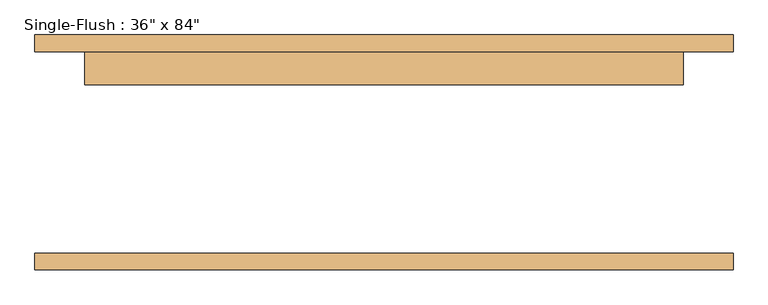
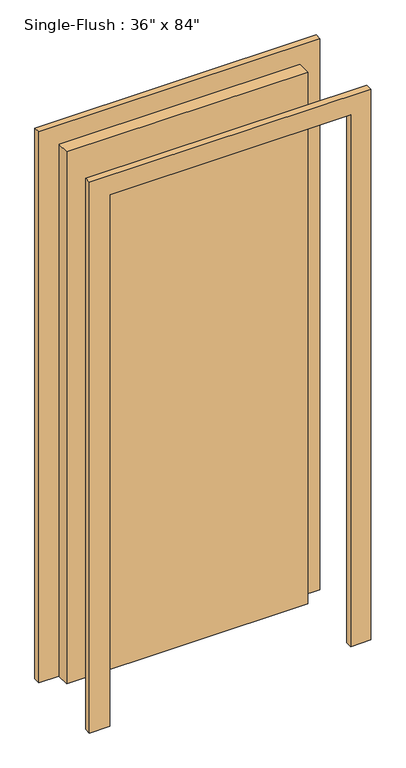
"""IFC4 building model written with IfcOpenShell, lengths in millimetres: door geometry."""

from ifc_helpers import new_model, si_unit, frame, origin, origin_with_axes, place, context, project, spatial, polyline, outline, extrude, source, transform, mapped, element, save


def door_4e13689c(model_context):
    return source(origin(), model_context, "Body", "SweptSolid", [
        extrude(outline(polyline([(2209.8, -533.4), (0.0, -533.4), (0.0, -457.2), (2133.6, -457.2), (2133.6, 457.2), (0.0, 457.2), (0.0, 533.4), (2209.8, 533.4), (2209.8, -533.4)])), frame((0.0, 153.9875, 0.0), z_axis=(0.0, 1.0, 0.0), x_axis=(0.0, 0.0, 1.0)), (0.0, 0.0, 1.0), 25.4),
        extrude(outline(polyline([(2209.8, 533.4), (2209.8, -533.4), (0.0, -533.4), (0.0, -457.2), (2133.6, -457.2), (2133.6, 457.2), (0.0, 457.2), (0.0, 533.4), (2209.8, 533.4)])), frame((0.0, -179.3875, 0.0), z_axis=(0.0, 1.0, 0.0), x_axis=(0.0, 0.0, 1.0)), (0.0, 0.0, 1.0), 25.4),
        extrude(outline(polyline([(457.2, 103.1875), (-457.2, 103.1875), (-457.2, 153.9875), (457.2, 153.9875), (457.2, 103.1875)])), origin_with_axes(), (0.0, 0.0, 1.0), 2133.6),
    ])


if __name__ == "__main__":
    model = new_model("IFC4")
    model_context = context("Model", 3, world=origin())
    ifc_project = project(units=[si_unit("LENGTHUNIT", "METRE", prefix="MILLI")], contexts=[model_context])
    site = spatial("IfcSite", under=ifc_project)
    building = spatial("IfcBuilding", under=site)
    placement = place(None, origin())
    door_shape = door_4e13689c(model_context)
    element("IfcDoor", 1, ObjectType="Single-Flush : 36\" x 84\"", at=placement, inside=building, context=model_context, shape_type="MappedRepresentation", body=[
        mapped(door_shape, transform((0.0, 0.0, 0.0), x_axis=(1.0, 0.0, 0.0), y_axis=(0.0, 1.0, 0.0), z_axis=(0.0, 0.0, 1.0))),
    ])
    save(model, "model.ifc")

# Revit data of these elements
# Type "Single-Flush : 36\" x 84\""
#   Type Mark = "1"
#   Assembly Code = "C1020"
#   Thickness = 0' - 2"
#   Height = 7' - 0"
#   Trim Projection Ext = 0' - 1"
#   Trim Projection Int = 0' - 1"
#   Trim Width = 0' - 3"
#   Width = 3' - 0"
#   Function = 0
#   Door Material = Door - Panel
#   Frame Material = Door - Frame
#   Wall Closure = (empty or 0)
# Element 1 (IfcDoor, "Single-Flush : 36\" x 84\"")
#   Materials on its faces: "Door - Frame", "Door - Panel"
# Materials
#   "Door - Panel": class "Wood", colour RGB 210 159 95, transparency 0
#   "Door - Frame": class "Miscellaneous", colour RGB 118 70 51, transparency 0
